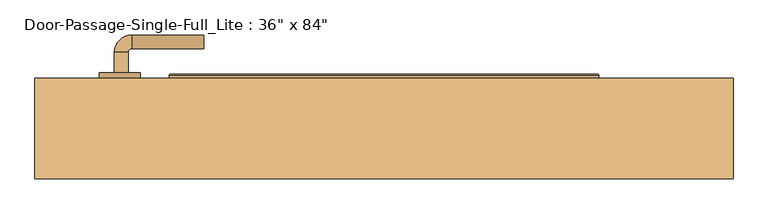
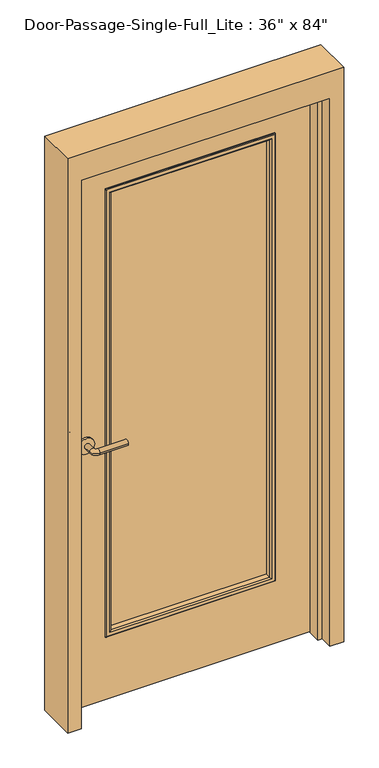
"""IFC4 building model written with IfcOpenShell, lengths in millimetres: door geometry."""

from ifc_helpers import new_model, si_unit, point, frame, frame_2d, origin, place, context, project, spatial, polyline, circle_curve, ellipse_curve, trimmed, segment, composite_curve, outline, extrude, faceted_brep, source, transform, mapped, element, save
from ifc_brep_helpers import plane_surface, cylinder_surface, revolved_surface, advanced_brep


def door_72024a31(model_context):
    return source(origin(), model_context, "Body", "SolidModel", [
        advanced_brep(
        [(-392.190625, -1.65, 1016.0), (-372.190625, -1.65, 1016.0), (-372.190625, -31.65, 1016.0), (-392.190625, -31.65, 1016.0), (-367.190625, -36.65, 1016.0), (-367.190625, -56.65, 1016.0), (-262.190625, -56.65, 1016.0), (-262.190625, -36.65, 1016.0)],
        [
            (0, 1, circle_curve(frame((-382.190625, -1.65, 1016.0), z_axis=(0.0, 1.0, 0.0), x_axis=(1.0, 0.0, 0.0)), 10.0)),
            (1, 0, circle_curve(frame((-382.190625, -1.65, 1016.0), z_axis=(0.0, 1.0, 0.0), x_axis=(1.0, 0.0, 0.0)), 10.0)),
            (1, 2),
            (2, 3, circle_curve(frame((-382.190625, -31.65, 1016.0), z_axis=(0.0, 1.0, 0.0), x_axis=(1.0, 0.0, 0.0)), 10.0)),
            (3, 0),
            (3, 2, circle_curve(frame((-382.190625, -31.65, 1016.0), z_axis=(0.0, 1.0, 0.0), x_axis=(1.0, 0.0, 0.0)), 10.0)),
            (4, 5, circle_curve(frame((-367.190625, -46.65, 1016.0), z_axis=(-1.0, 0.0, 0.0), x_axis=(0.0, 1.0, 0.0)), 10.0)),
            (5, 3, circle_curve(frame((-367.190625, -31.65, 1016.0), z_axis=(0.0, 0.0, -1.0), x_axis=(-1.0, 0.0, 0.0)), 25.0)),
            (2, 4, circle_curve(frame((-367.190625, -31.65, 1016.0), z_axis=(0.0, 0.0, 1.0), x_axis=(-1.0, 0.0, 0.0)), 5.0)),
            (5, 4, circle_curve(frame((-367.190625, -46.65, 1016.0), z_axis=(-1.0, 0.0, 0.0), x_axis=(0.0, 1.0, 0.0)), 10.0)),
            (6, 7, circle_curve(frame((-262.190625, -46.65, 1016.0), z_axis=(1.0, 0.0, 0.0), x_axis=(0.0, 1.0, 0.0)), 10.0)),
            (7, 6, circle_curve(frame((-262.190625, -46.65, 1016.0), z_axis=(1.0, 0.0, 0.0), x_axis=(0.0, 1.0, 0.0)), 10.0)),
            (4, 7),
            (6, 5),
        ],
        [
            plane_surface(frame((-382.190625, -1.65, 1016.0), z_axis=(0.0, 1.0, 0.0), x_axis=(0.0, 0.0, 1.0))),
            cylinder_surface(frame((-382.190625, -1.65, 1016.0), z_axis=(0.0, 1.0, 0.0), x_axis=(1.0, 0.0, 0.0)), 10.0),
            revolved_surface(trimmed(ellipse_curve(frame((-382.190625, -31.65, 1016.0), z_axis=(0.0, -1.0, 0.0), x_axis=(1.0, 0.0, 0.0)), 10.0, 10.0), [point((-392.190625, -31.65, 1016.0))], [point((-372.190625, -31.65, 1016.0))], True, "CARTESIAN"), (-367.190625, -31.65, 1016.0), (0.0, 0.0, -1.0)),
            revolved_surface(trimmed(ellipse_curve(frame((-382.190625, -31.65, 1016.0), z_axis=(0.0, -1.0, 0.0), x_axis=(1.0, 0.0, 0.0)), 10.0, 10.0), [point((-372.190625, -31.65, 1016.0))], [point((-392.190625, -31.65, 1016.0))], True, "CARTESIAN"), (-367.190625, -31.65, 1016.0), (0.0, 0.0, -1.0)),
            plane_surface(frame((-262.190625, -46.65, 1016.0), z_axis=(1.0, 0.0, 0.0), x_axis=(0.0, 0.0, 1.0))),
            cylinder_surface(frame((-367.190625, -46.65, 1016.0), z_axis=(-1.0, 0.0, 0.0), x_axis=(0.0, 1.0, 0.0)), 10.0),
        ],
        [
            (0, [[1, 2]]),
            (1, [[3, 4, 5, -2]]),
            (1, [[-5, 6, -3, -1]]),
            (2, [[7, 8, -4, 9]]),
            (3, [[10, -9, -6, -8]]),
            (4, [[11, 12]]),
            (5, [[13, -11, 14, -7]]),
            (5, [[-14, -12, -13, -10]]),
        ],
    ),
        extrude(outline(composite_curve([segment(trimmed(circle_curve(frame_2d((1016.0, -384.690625)), 30.0), [point((1016.0, -414.690625))], [point((1016.0, -354.690625))], False, "CARTESIAN"), True, "CONTINUOUS"), segment(trimmed(circle_curve(frame_2d((1016.0, -384.690625)), 30.0), [point((1016.0, -354.690625))], [point((1016.0, -414.690625))], False, "CARTESIAN"), True, "CONTINUOUS")], self_intersect=False)), frame((0.0, -1.65, 0.0), z_axis=(0.0, 1.0, 0.0), x_axis=(0.0, 0.0, 1.0)), (0.0, 0.0, 1.0), 8.0),
        advanced_brep(
        [(-392.190625, 58.8, 1016.0), (-372.190625, 58.8, 1016.0), (-392.190625, 88.8, 1016.0), (-372.190625, 88.8, 1016.0), (-367.190625, 93.8, 1016.0), (-367.190625, 113.8, 1016.0), (-262.190625, 113.8, 1016.0), (-262.190625, 93.8, 1016.0)],
        [
            (0, 1, circle_curve(frame((-382.190625, 58.8, 1016.0), z_axis=(0.0, -1.0, 0.0), x_axis=(1.0, 0.0, 0.0)), 10.0)),
            (1, 0, circle_curve(frame((-382.190625, 58.8, 1016.0), z_axis=(0.0, -1.0, 0.0), x_axis=(1.0, 0.0, 0.0)), 10.0)),
            (0, 2),
            (2, 3, circle_curve(frame((-382.190625, 88.8, 1016.0), z_axis=(0.0, -1.0, 0.0), x_axis=(1.0, 0.0, 0.0)), 10.0)),
            (3, 1),
            (3, 2, circle_curve(frame((-382.190625, 88.8, 1016.0), z_axis=(0.0, -1.0, 0.0), x_axis=(1.0, 0.0, 0.0)), 10.0)),
            (4, 3, circle_curve(frame((-367.190625, 88.8, 1016.0), z_axis=(0.0, 0.0, 1.0), x_axis=(-1.0, 0.0, 0.0)), 5.0)),
            (2, 5, circle_curve(frame((-367.190625, 88.8, 1016.0), z_axis=(0.0, 0.0, -1.0), x_axis=(-1.0, 0.0, 0.0)), 25.0)),
            (5, 4, circle_curve(frame((-367.190625, 103.8, 1016.0), z_axis=(-1.0, 0.0, 0.0), x_axis=(0.0, -1.0, 0.0)), 10.0)),
            (4, 5, circle_curve(frame((-367.190625, 103.8, 1016.0), z_axis=(-1.0, 0.0, 0.0), x_axis=(0.0, -1.0, 0.0)), 10.0)),
            (6, 7, circle_curve(frame((-262.190625, 103.8, 1016.0), z_axis=(1.0, 0.0, 0.0), x_axis=(0.0, -1.0, 0.0)), 10.0)),
            (7, 6, circle_curve(frame((-262.190625, 103.8, 1016.0), z_axis=(1.0, 0.0, 0.0), x_axis=(0.0, -1.0, 0.0)), 10.0)),
            (5, 6),
            (7, 4),
        ],
        [
            plane_surface(frame((-382.190625, 58.8, 1016.0), z_axis=(0.0, -1.0, 0.0), x_axis=(0.0, 0.0, 1.0))),
            cylinder_surface(frame((-382.190625, 58.8, 1016.0), z_axis=(0.0, -1.0, 0.0), x_axis=(1.0, 0.0, 0.0)), 10.0),
            revolved_surface(trimmed(ellipse_curve(frame((-382.190625, 88.8, 1016.0), z_axis=(0.0, -1.0, 0.0), x_axis=(1.0, 0.0, 0.0)), 10.0, 10.0), [point((-392.190625, 88.8, 1016.0))], [point((-372.190625, 88.8, 1016.0))], True, "CARTESIAN"), (-367.190625, 88.8, 1016.0), (0.0, 0.0, -1.0)),
            revolved_surface(trimmed(ellipse_curve(frame((-382.190625, 88.8, 1016.0), z_axis=(0.0, -1.0, 0.0), x_axis=(1.0, 0.0, 0.0)), 10.0, 10.0), [point((-372.190625, 88.8, 1016.0))], [point((-392.190625, 88.8, 1016.0))], True, "CARTESIAN"), (-367.190625, 88.8, 1016.0), (0.0, 0.0, -1.0)),
            plane_surface(frame((-262.190625, 103.8, 1016.0), z_axis=(1.0, 0.0, 0.0), x_axis=(0.0, 0.0, 1.0))),
            cylinder_surface(frame((-367.190625, 103.8, 1016.0), z_axis=(-1.0, 0.0, 0.0), x_axis=(0.0, -1.0, 0.0)), 10.0),
        ],
        [
            (0, [[1, 2]]),
            (1, [[-1, 3, 4, 5]]),
            (1, [[-2, -5, 6, -3]]),
            (2, [[7, -4, 8, 9]]),
            (3, [[-8, -6, -7, 10]]),
            (4, [[11, 12]]),
            (5, [[-9, 13, -12, 14]]),
            (5, [[-10, -14, -11, -13]]),
        ],
    ),
        extrude(outline(composite_curve([segment(trimmed(circle_curve(frame_2d((1016.0, -384.690625)), 30.0), [point((1016.0, -414.690625))], [point((1016.0, -354.690625))], False, "CARTESIAN"), True, "CONTINUOUS"), segment(trimmed(circle_curve(frame_2d((1016.0, -384.690625)), 30.0), [point((1016.0, -354.690625))], [point((1016.0, -414.690625))], False, "CARTESIAN"), True, "CONTINUOUS")], self_intersect=False)), frame((0.0, 50.8, 0.0), z_axis=(0.0, 1.0, 0.0), x_axis=(0.0, 0.0, 1.0)), (0.0, 0.0, 1.0), 8.0),
        extrude(outline(polyline([(304.8, 25.4), (-304.8, 25.4), (-304.8, 31.75), (304.8, 31.75), (304.8, 25.4)])), frame((0.0, 0.0, 254.0), z_axis=(0.0, 0.0, 1.0), x_axis=(1.0, 0.0, 0.0)), (0.0, 0.0, 1.0), 1727.2),
        faceted_brep([(457.2, 1.5875, 0.0), (457.2, 50.8, 0.0), (508.0, 50.8, 0.0), (508.0, -95.25, 0.0), (457.2, -95.25, 0.0), (457.2, -46.0375, 0.0), (441.325, -46.0375, 0.0), (441.325, 1.5875, 0.0), (457.2, 1.5875, 2133.6), (457.2, 50.8, 2133.6), (-457.2, 50.8, 2133.6), (-457.2, 50.8, 0.0), (-508.0, 50.8, 0.0), (-508.0, 50.8, 2235.2), (508.0, 50.8, 2235.2), (508.0, -95.25, 2235.2), (-508.0, -95.25, 2235.2), (-508.0, -95.25, 0.0), (-457.2, -95.25, 0.0), (-457.2, -95.25, 2133.6), (457.2, -95.25, 2133.6), (457.2, -46.0375, 2133.6), (-457.2, -46.0375, 2133.6), (-457.2, -46.0375, 0.0), (-441.325, -46.0375, 0.0), (-441.325, -46.0375, 2117.725), (441.325, -46.0375, 2117.725), (441.325, 1.5875, 2117.725), (-441.325, 1.5875, 2117.725), (-441.325, 1.5875, 0.0), (-457.2, 1.5875, 0.0), (-457.2, 1.5875, 2133.6)], [[[0, 1, 2, 3, 4, 5, 6, 7]], [[1, 0, 8, 9]], [[2, 1, 9, 10, 11, 12, 13, 14]], [[3, 2, 14, 15]], [[4, 3, 15, 16, 17, 18, 19, 20]], [[5, 4, 20, 21]], [[6, 5, 21, 22, 23, 24, 25, 26]], [[7, 6, 26, 27]], [[0, 7, 27, 28, 29, 30, 31, 8]], [[9, 8, 31, 10]], [[20, 19, 22, 21]], [[26, 25, 28, 27]], [[12, 11, 30, 29, 24, 23, 18, 17]], [[11, 10, 31, 30]], [[13, 12, 17, 16]], [[19, 18, 23, 22]], [[25, 24, 29, 28]], [[15, 14, 13, 16]]]),
        extrude(outline(polyline([(2133.6, -457.2), (0.0, -457.2), (0.0, 457.2), (2133.6, 457.2), (2133.6, -457.2)]), holes=[polyline([(1981.2, -304.8), (1981.2, 304.8), (254.0, 304.8), (254.0, -304.8), (1981.2, -304.8)])]), frame((0.0, 6.35, 0.0), z_axis=(0.0, 1.0, 0.0), x_axis=(0.0, 0.0, 1.0)), (0.0, 0.0, 1.0), 44.45),
        advanced_brep(
        [(-304.8, 31.75, 1981.2), (-304.8, 50.8, 1981.2), (-304.8, 50.8, 254.0), (-304.8, 31.75, 254.0), (-292.8, 51.8, 1969.2), (-292.8, 31.75, 1969.2), (-292.8, 31.75, 266.0), (-292.8, 51.8, 266.0), (-297.8, 56.8, 1974.2), (-297.8, 56.8, 261.0), (-312.8, 54.8, 1989.2), (-310.8, 56.8, 1987.2), (-310.8, 56.8, 248.0), (-312.8, 54.8, 246.0), (-312.8, 50.8, 1989.2), (-312.8, 50.8, 246.0), (304.8, 50.8, 254.0), (304.8, 31.75, 254.0), (292.8, 31.75, 266.0), (292.8, 51.8, 266.0), (297.8, 56.8, 261.0), (310.8, 56.8, 248.0), (312.8, 54.8, 246.0), (312.8, 50.8, 246.0), (304.8, 50.8, 1981.2), (304.8, 31.75, 1981.2), (292.8, 31.75, 1969.2), (292.8, 51.8, 1969.2), (297.8, 56.8, 1974.2), (310.8, 56.8, 1987.2), (312.8, 54.8, 1989.2), (312.8, 50.8, 1989.2)],
        [
            (0, 1),
            (1, 2),
            (2, 3),
            (3, 0),
            (4, 5),
            (5, 6),
            (6, 7),
            (7, 4),
            (8, 4, ellipse_curve(frame((-297.8, 51.8, 1974.2), z_axis=(-0.7071067811865475, 0.0, -0.7071067811865475), x_axis=(-0.7071067811865474, 0.0, 0.7071067811865476)), 7.0710678, 5.0)),
            (7, 9, ellipse_curve(frame((-297.8, 51.8, 261.0), z_axis=(-0.7071067811865475, 0.0, 0.7071067811865475), x_axis=(0.7071067811865474, 0.0, 0.7071067811865476)), 7.0710678, 5.0)),
            (9, 8),
            (10, 11, ellipse_curve(frame((-310.8, 54.8, 1987.2), z_axis=(-0.7071067811865475, 0.0, -0.7071067811865475), x_axis=(-0.7071067811865474, 0.0, 0.7071067811865476)), 2.8284271, 2.0)),
            (11, 12),
            (12, 13, ellipse_curve(frame((-310.8, 54.8, 248.0), z_axis=(-0.7071067811865475, 0.0, 0.7071067811865475), x_axis=(0.7071067811865474, 0.0, 0.7071067811865476)), 2.8284271, 2.0)),
            (13, 10),
            (14, 10),
            (13, 15),
            (15, 14),
            (2, 16),
            (16, 17),
            (17, 3),
            (6, 18),
            (18, 19),
            (19, 7),
            (19, 20, ellipse_curve(frame((297.8, 51.8, 261.0), z_axis=(-0.7071067811865475, 0.0, -0.7071067811865475), x_axis=(-0.7071067811865476, 0.0, 0.7071067811865474)), 7.0710678, 5.0)),
            (20, 9),
            (12, 21),
            (21, 22, ellipse_curve(frame((310.8, 54.8, 248.0), z_axis=(-0.7071067811865475, 0.0, -0.7071067811865475), x_axis=(-0.7071067811865476, 0.0, 0.7071067811865474)), 2.8284271, 2.0)),
            (22, 13),
            (22, 23),
            (23, 15),
            (16, 24),
            (24, 25),
            (25, 17),
            (18, 26),
            (26, 27),
            (27, 19),
            (27, 28, ellipse_curve(frame((297.8, 51.8, 1974.2), z_axis=(0.7071067811865475, 0.0, -0.7071067811865475), x_axis=(-0.7071067811865474, 0.0, -0.7071067811865476)), 7.0710678, 5.0)),
            (28, 20),
            (21, 29),
            (29, 30, ellipse_curve(frame((310.8, 54.8, 1987.2), z_axis=(0.7071067811865475, 0.0, -0.7071067811865475), x_axis=(-0.7071067811865474, 0.0, -0.7071067811865476)), 2.8284271, 2.0)),
            (30, 22),
            (30, 31),
            (31, 23),
            (31, 14),
            (1, 24),
            (0, 25),
            (5, 26),
            (4, 27),
            (8, 28),
            (11, 29),
            (10, 30),
        ],
        [
            plane_surface(frame((-304.8, 50.8, 1981.2), z_axis=(-1.0, 0.0, 0.0), x_axis=(0.0, 0.0, -1.0))),
            plane_surface(frame((-292.8, 31.75, 1969.2), z_axis=(1.0, 0.0, 0.0), x_axis=(0.0, 0.0, -1.0))),
            cylinder_surface(frame((-297.8, 51.8, 1981.2), z_axis=(0.0, 0.0, 1.0), x_axis=(-1.0, 0.0, 0.0)), 5.0),
            cylinder_surface(frame((-310.8, 54.8, 1981.2), z_axis=(0.0, 0.0, 1.0), x_axis=(-1.0, 0.0, 0.0)), 2.0),
            plane_surface(frame((-312.8, 54.8, 1989.2), z_axis=(-1.0, 0.0, 0.0), x_axis=(0.0, 0.0, -1.0))),
            plane_surface(frame((-304.8, 50.8, 254.0), z_axis=(0.0, 0.0, -1.0), x_axis=(1.0, 0.0, 0.0))),
            plane_surface(frame((-292.8, 31.75, 266.0), z_axis=(0.0, 0.0, 1.0), x_axis=(1.0, 0.0, 0.0))),
            cylinder_surface(frame((-304.8, 51.8, 261.0), z_axis=(-1.0, 0.0, 0.0), x_axis=(0.0, 0.0, -1.0)), 5.0),
            cylinder_surface(frame((-304.8, 54.8, 248.0), z_axis=(-1.0, 0.0, 0.0), x_axis=(0.0, 0.0, -1.0)), 2.0),
            plane_surface(frame((-312.8, 54.8, 246.0), z_axis=(0.0, 0.0, -1.0), x_axis=(1.0, 0.0, 0.0))),
            plane_surface(frame((304.8, 50.8, 254.0), z_axis=(1.0, 0.0, 0.0), x_axis=(0.0, 0.0, 1.0))),
            plane_surface(frame((292.8, 31.75, 266.0), z_axis=(-1.0, 0.0, 0.0), x_axis=(0.0, 0.0, 1.0))),
            cylinder_surface(frame((297.8, 51.8, 254.0), z_axis=(0.0, 0.0, -1.0), x_axis=(1.0, 0.0, 0.0)), 5.0),
            cylinder_surface(frame((310.8, 54.8, 254.0), z_axis=(0.0, 0.0, -1.0), x_axis=(1.0, 0.0, 0.0)), 2.0),
            plane_surface(frame((312.8, 54.8, 246.0), z_axis=(1.0, 0.0, 0.0), x_axis=(0.0, 0.0, 1.0))),
            plane_surface(frame((312.8, 50.8, 1989.2), z_axis=(0.0, -1.0, 0.0), x_axis=(-1.0, 0.0, 0.0))),
            plane_surface(frame((304.8, 50.8, 1981.2), z_axis=(0.0, 0.0, 1.0), x_axis=(-1.0, 0.0, 0.0))),
            plane_surface(frame((304.8, 31.75, 1981.2), z_axis=(0.0, -1.0, 0.0), x_axis=(-1.0, 0.0, 0.0))),
            plane_surface(frame((292.8, 31.75, 1969.2), z_axis=(0.0, 0.0, -1.0), x_axis=(-1.0, 0.0, 0.0))),
            cylinder_surface(frame((304.8, 51.8, 1974.2), z_axis=(1.0, 0.0, 0.0), x_axis=(0.0, 0.0, 1.0)), 5.0),
            plane_surface(frame((297.8, 56.8, 1974.2), z_axis=(0.0, 1.0, 0.0), x_axis=(-1.0, 0.0, 0.0))),
            cylinder_surface(frame((304.8, 54.8, 1987.2), z_axis=(1.0, 0.0, 0.0), x_axis=(0.0, 0.0, 1.0)), 2.0),
            plane_surface(frame((312.8, 54.8, 1989.2), z_axis=(0.0, 0.0, 1.0), x_axis=(-1.0, 0.0, 0.0))),
        ],
        [
            (0, [[1, 2, 3, 4]]),
            (1, [[5, 6, 7, 8]]),
            (2, [[9, -8, 10, 11]]),
            (3, [[12, 13, 14, 15]]),
            (4, [[16, -15, 17, 18]]),
            (5, [[-3, 19, 20, 21]]),
            (6, [[-7, 22, 23, 24]]),
            (7, [[-10, -24, 25, 26]]),
            (8, [[-14, 27, 28, 29]]),
            (9, [[-17, -29, 30, 31]]),
            (10, [[-20, 32, 33, 34]]),
            (11, [[-23, 35, 36, 37]]),
            (12, [[-25, -37, 38, 39]]),
            (13, [[-28, 40, 41, 42]]),
            (14, [[-30, -42, 43, 44]]),
            (15, [[-31, -44, 45, -18], [46, -32, -19, -2]]),
            (16, [[-33, -46, -1, 47]]),
            (17, [[-21, -34, -47, -4], [48, -35, -22, -6]]),
            (18, [[-36, -48, -5, 49]]),
            (19, [[-38, -49, -9, 50]]),
            (20, [[51, -40, -27, -13], [-26, -39, -50, -11]]),
            (21, [[-41, -51, -12, 52]]),
            (22, [[-43, -52, -16, -45]]),
        ],
    ),
        advanced_brep(
        [(-304.8, 25.4, 254.0), (-304.8, 6.35, 254.0), (-304.8, 6.35, 1981.2), (-304.8, 25.4, 1981.2), (-292.8, 5.35, 266.0), (-292.8, 25.4, 266.0), (-292.8, 25.4, 1969.2), (-292.8, 5.35, 1969.2), (-297.8, 0.35, 261.0), (-297.8, 0.35, 1974.2), (-312.8, 2.35, 246.0), (-310.8, 0.35, 248.0), (-310.8, 0.35, 1987.2), (-312.8, 2.35, 1989.2), (-312.8, 6.35, 246.0), (-312.8, 6.35, 1989.2), (304.8, 6.35, 1981.2), (304.8, 25.4, 1981.2), (292.8, 25.4, 1969.2), (292.8, 5.35, 1969.2), (297.8, 0.35, 1974.2), (310.8, 0.35, 1987.2), (312.8, 2.35, 1989.2), (312.8, 6.35, 1989.2), (304.8, 6.35, 254.0), (304.8, 25.4, 254.0), (292.8, 25.4, 266.0), (292.8, 5.35, 266.0), (297.8, 0.35, 261.0), (310.8, 0.35, 248.0), (312.8, 2.35, 246.0), (312.8, 6.35, 246.0)],
        [
            (0, 1),
            (1, 2),
            (2, 3),
            (3, 0),
            (4, 5),
            (5, 6),
            (6, 7),
            (7, 4),
            (8, 4, ellipse_curve(frame((-297.8, 5.35, 261.0), z_axis=(-0.7071067811865475, 0.0, 0.7071067811865475), x_axis=(-0.7071067811865474, 0.0, -0.7071067811865476)), 7.0710678, 5.0)),
            (7, 9, ellipse_curve(frame((-297.8, 5.35, 1974.2), z_axis=(-0.7071067811865475, 0.0, -0.7071067811865475), x_axis=(0.7071067811865474, 0.0, -0.7071067811865476)), 7.0710678, 5.0)),
            (9, 8),
            (10, 11, ellipse_curve(frame((-310.8, 2.35, 248.0), z_axis=(-0.7071067811865475, 0.0, 0.7071067811865475), x_axis=(-0.7071067811865474, 0.0, -0.7071067811865476)), 2.8284271, 2.0)),
            (11, 12),
            (12, 13, ellipse_curve(frame((-310.8, 2.35, 1987.2), z_axis=(-0.7071067811865475, 0.0, -0.7071067811865475), x_axis=(0.7071067811865474, 0.0, -0.7071067811865476)), 2.8284271, 2.0)),
            (13, 10),
            (14, 10),
            (13, 15),
            (15, 14),
            (2, 16),
            (16, 17),
            (17, 3),
            (6, 18),
            (18, 19),
            (19, 7),
            (19, 20, ellipse_curve(frame((297.8, 5.35, 1974.2), z_axis=(-0.7071067811865475, 0.0, 0.7071067811865475), x_axis=(-0.7071067811865476, 0.0, -0.7071067811865474)), 7.0710678, 5.0)),
            (20, 9),
            (12, 21),
            (21, 22, ellipse_curve(frame((310.8, 2.35, 1987.2), z_axis=(-0.7071067811865475, 0.0, 0.7071067811865475), x_axis=(-0.7071067811865476, 0.0, -0.7071067811865474)), 2.8284271, 2.0)),
            (22, 13),
            (22, 23),
            (23, 15),
            (16, 24),
            (24, 25),
            (25, 17),
            (18, 26),
            (26, 27),
            (27, 19),
            (27, 28, ellipse_curve(frame((297.8, 5.35, 261.0), z_axis=(0.7071067811865475, 0.0, 0.7071067811865475), x_axis=(-0.7071067811865474, 0.0, 0.7071067811865476)), 7.0710678, 5.0)),
            (28, 20),
            (21, 29),
            (29, 30, ellipse_curve(frame((310.8, 2.35, 248.0), z_axis=(0.7071067811865475, 0.0, 0.7071067811865475), x_axis=(-0.7071067811865474, 0.0, 0.7071067811865476)), 2.8284271, 2.0)),
            (30, 22),
            (30, 31),
            (31, 23),
            (31, 14),
            (1, 24),
            (0, 25),
            (5, 26),
            (4, 27),
            (8, 28),
            (11, 29),
            (10, 30),
        ],
        [
            plane_surface(frame((-304.8, 6.35, 254.0), z_axis=(-1.0, 0.0, 0.0), x_axis=(0.0, 0.0, 1.0))),
            plane_surface(frame((-292.8, 25.4, 266.0), z_axis=(1.0, 0.0, 0.0), x_axis=(0.0, 0.0, 1.0))),
            cylinder_surface(frame((-297.8, 5.35, 254.0), z_axis=(0.0, 0.0, -1.0), x_axis=(-1.0, 0.0, 0.0)), 5.0),
            cylinder_surface(frame((-310.8, 2.35, 254.0), z_axis=(0.0, 0.0, -1.0), x_axis=(-1.0, 0.0, 0.0)), 2.0),
            plane_surface(frame((-312.8, 2.35, 246.0), z_axis=(-1.0, 0.0, 0.0), x_axis=(0.0, 0.0, 1.0))),
            plane_surface(frame((-304.8, 6.35, 1981.2), z_axis=(0.0, 0.0, 1.0), x_axis=(1.0, 0.0, 0.0))),
            plane_surface(frame((-292.8, 25.4, 1969.2), z_axis=(0.0, 0.0, -1.0), x_axis=(1.0, 0.0, 0.0))),
            cylinder_surface(frame((-304.8, 5.35, 1974.2), z_axis=(-1.0, 0.0, 0.0), x_axis=(0.0, 0.0, 1.0)), 5.0),
            cylinder_surface(frame((-304.8, 2.35, 1987.2), z_axis=(-1.0, 0.0, 0.0), x_axis=(0.0, 0.0, 1.0)), 2.0),
            plane_surface(frame((-312.8, 2.35, 1989.2), z_axis=(0.0, 0.0, 1.0), x_axis=(1.0, 0.0, 0.0))),
            plane_surface(frame((304.8, 6.35, 1981.2), z_axis=(1.0, 0.0, 0.0), x_axis=(0.0, 0.0, -1.0))),
            plane_surface(frame((292.8, 25.4, 1969.2), z_axis=(-1.0, 0.0, 0.0), x_axis=(0.0, 0.0, -1.0))),
            cylinder_surface(frame((297.8, 5.35, 1981.2), z_axis=(0.0, 0.0, 1.0), x_axis=(1.0, 0.0, 0.0)), 5.0),
            cylinder_surface(frame((310.8, 2.35, 1981.2), z_axis=(0.0, 0.0, 1.0), x_axis=(1.0, 0.0, 0.0)), 2.0),
            plane_surface(frame((312.8, 2.35, 1989.2), z_axis=(1.0, 0.0, 0.0), x_axis=(0.0, 0.0, -1.0))),
            plane_surface(frame((312.8, 6.35, 246.0), z_axis=(0.0, 1.0, 0.0), x_axis=(-1.0, 0.0, 0.0))),
            plane_surface(frame((304.8, 6.35, 254.0), z_axis=(0.0, 0.0, -1.0), x_axis=(-1.0, 0.0, 0.0))),
            plane_surface(frame((304.8, 25.4, 254.0), z_axis=(0.0, 1.0, 0.0), x_axis=(-1.0, 0.0, 0.0))),
            plane_surface(frame((292.8, 25.4, 266.0), z_axis=(0.0, 0.0, 1.0), x_axis=(-1.0, 0.0, 0.0))),
            cylinder_surface(frame((304.8, 5.35, 261.0), z_axis=(1.0, 0.0, 0.0), x_axis=(0.0, 0.0, -1.0)), 5.0),
            plane_surface(frame((297.8, 0.35, 261.0), z_axis=(0.0, -1.0, 0.0), x_axis=(-1.0, 0.0, 0.0))),
            cylinder_surface(frame((304.8, 2.35, 248.0), z_axis=(1.0, 0.0, 0.0), x_axis=(0.0, 0.0, -1.0)), 2.0),
            plane_surface(frame((312.8, 2.35, 246.0), z_axis=(0.0, 0.0, -1.0), x_axis=(-1.0, 0.0, 0.0))),
        ],
        [
            (0, [[1, 2, 3, 4]]),
            (1, [[5, 6, 7, 8]]),
            (2, [[9, -8, 10, 11]]),
            (3, [[12, 13, 14, 15]]),
            (4, [[16, -15, 17, 18]]),
            (5, [[-3, 19, 20, 21]]),
            (6, [[-7, 22, 23, 24]]),
            (7, [[-10, -24, 25, 26]]),
            (8, [[-14, 27, 28, 29]]),
            (9, [[-17, -29, 30, 31]]),
            (10, [[-20, 32, 33, 34]]),
            (11, [[-23, 35, 36, 37]]),
            (12, [[-25, -37, 38, 39]]),
            (13, [[-28, 40, 41, 42]]),
            (14, [[-30, -42, 43, 44]]),
            (15, [[-31, -44, 45, -18], [46, -32, -19, -2]]),
            (16, [[-33, -46, -1, 47]]),
            (17, [[-21, -34, -47, -4], [48, -35, -22, -6]]),
            (18, [[-36, -48, -5, 49]]),
            (19, [[-38, -49, -9, 50]]),
            (20, [[51, -40, -27, -13], [-26, -39, -50, -11]]),
            (21, [[-41, -51, -12, 52]]),
            (22, [[-43, -52, -16, -45]]),
        ],
    ),
    ])


if __name__ == "__main__":
    model = new_model("IFC4")
    model_context = context("Model", 3, world=origin())
    ifc_project = project(units=[si_unit("LENGTHUNIT", "METRE", prefix="MILLI")], contexts=[model_context])
    site = spatial("IfcSite", under=ifc_project)
    building = spatial("IfcBuilding", under=site)
    placement = place(None, origin())
    door_shape = door_72024a31(model_context)
    element("IfcDoor", 1, ObjectType="Door-Passage-Single-Full_Lite : 36\" x 84\"", at=placement, inside=building, context=model_context, shape_type="MappedRepresentation", body=[
        mapped(door_shape, transform((0.0, 0.0, 0.0), x_axis=(1.0, 0.0, 0.0), y_axis=(0.0, 1.0, 0.0), z_axis=(0.0, 0.0, 1.0))),
    ])
    save(model, "model.ifc")

# Revit data of these elements
# Type "Door-Passage-Single-Full_Lite : 36\" x 84\""
#   Type Mark = "52"
#   Assembly Code = "B2030100"
#   Analytic Construction = "Wooden"
#   Thickness = 0' - 1 3/4"
#   Thermal Resistance (R) = 2.5876 (h·ft²·°F)/BTU
#   Swing Angle [instance default] = 90.00°
#   Strike Height = 3' - 4"
#   Rough Width [instance default] = 3' - 4"
#   Rough Height [instance default] = 7' - 4"
#   MF Opening Height [instance default] = 0' - 4"
#   MF Opening Width [instance default] = 0' - 4"
#   Inset Calculate [instance default] = 0' - 4"
#   Masonry Inset [instance default] = 0' - 1"
#   Height = 7' - 0"
#   Width = 3' - 0"
#   Heat Transfer Coefficient (U) = 0.3865 BTU/(h·ft²·°F)
#   Masonry Frame Depth = 0' - 5 3/4"
#   Masonry Frame [instance default] = yes
#   Function = 1
#   Dry Wall Frame [instance default] = no
#   Panel Material = Wood - Birch
#   Glazing = Glass
#   Glass Stop Material = Metal - Paint Finish - Grey
#   Frame Material = Metal - Paint Finish - Grey
#   Door Handle Material = Aluminum
#   Visual Light Transmittance = 0
#   Solar Heat Gain Coefficient = 0
#   Wall Closure = (empty or 0)
# Element 1 (IfcDoor, "Door-Passage-Single-Full_Lite : 36\" x 84\"")
#   Materials on its faces: "Metal - Paint Finish - Grey", "Aluminum", "Wood - Birch", "Glass"
# Materials
#   "Wood - Birch": class "Wood", colour RGB 166 116 52, transparency 0, Cost = 0
#   "Glass": class "Glass", colour RGB 0 128 192, transparency 0.75, Description = "Soda Lime Glass", Cost = 0
#   "Metal - Paint Finish - Grey": class "Paint", colour RGB 104 104 104, transparency 0, Cost = 0
#   "Aluminum": class "Metal", colour RGB 247 247 247, transparency 0, Description = "Aluminum 6061", Cost = 0
